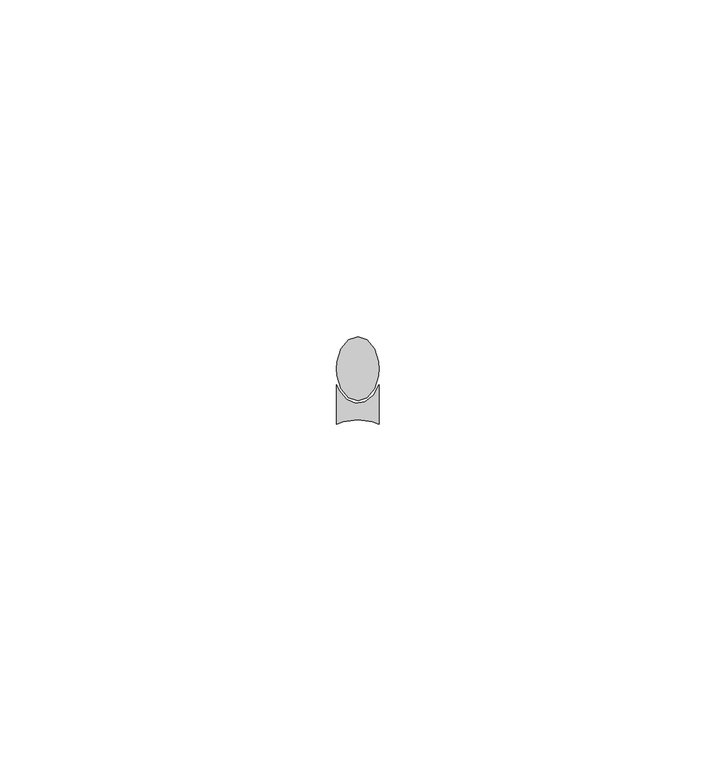
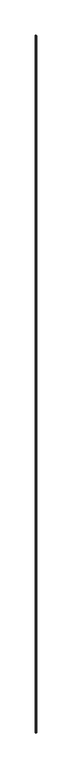
"""IFC4 building model written with IfcOpenShell, lengths in millimetres: proxy geometry, Generic Models 11:Generic Models 1:306267:Generic Models 1:306267 : Generic Models 11:Generic Models 1:306267:300405:Generic Models 1:306267:Generic Models 1:306267 : Generic Models 11:Generic Models 1:306267:300405 : Generic Models 11:Generic Models 1:306267:Generic Models 1:306267 : Generic Models 11:Generic Models 1:306267:300405:13 : Generic Models 11:Generic Models 1:306267:Generic Models 1:306267 : Generic Models 11:Generic Models 1:306267:300405:Generic Models 1:306267:Generic Models 1:306267 : Generic Models 11:Generic Models 1:306267:300405 : Generic Models 11:Generic Models 1:306267:Generic Models 1:306267 : Generic Models 11:Generic Models 1:306267:300405:300182."""

from ifc_helpers import new_model, si_unit, origin, origin_with_axes, place, context, project, spatial, polyline, outline, extrude, source, transform, mapped, element, save


def generic_models_64d3e4db(model_context):
    return source(origin(), model_context, "Body", "SweptSolid", [
        extrude(outline(polyline([(593733.5341431, -579092.0005286), (593732.429409, -579090.6790346), (593731.8163278, -579088.7694203), (593731.7367239, -579087.7096644), (593731.8163278, -579086.6499084), (593732.429409, -579084.7402942), (593733.5341431, -579083.4188002), (593734.9117239, -579082.9471644), (593736.2893048, -579083.4188002), (593737.3940389, -579084.7402942), (593738.0071201, -579086.6499084), (593738.0867239, -579087.7096644), (593738.0071201, -579088.7694203), (593737.3940389, -579090.6790346), (593736.2893048, -579092.0005286), (593734.9117239, -579092.4721644), (593733.5341431, -579092.0005286)])), origin_with_axes(), (0.0, 0.0, 1.0), 6064.4581746),
        extrude(outline(polyline([(593737.1209607, -579095.5639755), (593734.9117239, -579095.2502894), (593732.7024872, -579095.5639755), (593731.7367239, -579095.9413841), (593731.7367239, -579090.073292), (593732.1230415, -579090.9335729), (593733.206527, -579092.2431481), (593734.5567747, -579092.8435016), (593735.962551, -579092.6407137), (593737.2039351, -579091.6665087), (593738.0867239, -579090.073292), (593738.0867239, -579095.9413841), (593737.1209607, -579095.5639755)])), origin_with_axes(), (0.0, 0.0, 1.0), 6062.9878028),
    ])


if __name__ == "__main__":
    model = new_model("IFC4")
    model_context = context("Model", 3, world=origin())
    ifc_project = project(units=[si_unit("LENGTHUNIT", "METRE", prefix="MILLI")], contexts=[model_context])
    site = spatial("IfcSite", under=ifc_project)
    building = spatial("IfcBuilding", under=site)
    placement = place(None, origin())
    generic_models_shape = generic_models_64d3e4db(model_context)
    element("IfcBuildingElementProxy", 1, Name="Generic Models 11:Generic Models 1:306267:Generic Models 1:306267 : Generic Models 11:Generic Models 1:306267:300405:Generic Models 1:306267:Generic Models 1:306267 : Generic Models 11:Generic Models 1:306267:300405 : Generic Models 11:Generic Models 1:306267:Generic Models 1:306267 : Generic Models 11:Generic Models 1:306267:300405:13 : Generic Models 11:Generic Models 1:306267:Generic Models 1:306267 : Generic Models 11:Generic Models 1:306267:300405:Generic Models 1:306267:Generic Models 1:306267 : Generic Models 11:Generic Models 1:306267:300405 : Generic Models 11:Generic Models 1:306267:Generic Models 1:306267 : Generic Models 11:Generic Models 1:306267:300405:300182", ObjectType="Generic Models 11:Generic Models 1:306267:Generic Models 1:306267 : Generic Models 11:Generic Models 1:306267:300405:Generic Models 1:306267:Generic Models 1:306267 : Generic Models 11:Generic Models 1:306267:300405 : Generic Models 11:Generic Models 1:306267:Generic Models 1:306267 : Generic Models 11:Generic Models 1:306267:300405:13 : Generic Models 11:Generic Models 1:306267:Generic Models 1:306267 : Generic Models 11:Generic Models 1:306267:300405:Generic Models 1:306267:Generic Models 1:306267 : Generic Models 11:Generic Models 1:306267:300405 : Generic Models 11:Generic Models 1:306267:Generic Models 1:306267 : Generic Models 11:Generic Models 1:306267:300405:300182", at=placement, inside=building, context=model_context, shape_type="MappedRepresentation", body=[
        mapped(generic_models_shape, transform((0.0, 0.0, 0.0), x_axis=(1.0, 0.0, 0.0), y_axis=(0.0, 1.0, 0.0), z_axis=(0.0, 0.0, 1.0))),
    ])
    save(model, "model.ifc")

# Revit data of these elements
# Type "Generic Models 11:Generic Models 1:306267:Generic Models 1:306267 : Generic Models 11:Generic Models 1:306267:300405:Generic Models 1:306267:Generic Models 1:306267 : Generic Models 11:Generic Models 1:306267:300405 : Generic Models 11:Generic Models 1:306267:Generic Models 1:306267 : Generic Models 11:Generic Models 1:306267:300405:13 : Generic Models 11:Generic Models 1:306267:Generic Models 1:306267 : Generic Models 11:Generic Models 1:306267:300405:Generic Models 1:306267:Generic Models 1:306267 : Generic Models 11:Generic Models 1:306267:300405 : Generic Models 11:Generic Models 1:306267:Generic Models 1:306267 : Generic Models 11:Generic Models 1:306267:300405:300182"
#   NameOverride = "Generic Models 11:Generic Models 1:306267:Generic Models 1:306267 : Generic Models 11:Generic Models 1:306267:300405:Generic Models 1:306267:Generic Models 1:306267 : Generic Models 11:Generic Models 1:306267:300405 : Generic Models 11:Generic Models 1:306267:Generic Models 1:306267 : Generic Models 11:Generic Models 1:306267:300405:300182"
#   ObjectTypeOverride = "Generic Models 1:306267:Generic Models 1:306267 : Generic Models 11:Generic Models 1:306267:300405 : Generic Models 11:Generic Models 1:306267:Generic Models 1:306267 : Generic Models 11:Generic Models 1:306267:300405"
#   Reference = "Generic Models 1"
#   Tag = "300182"
# Element 1 (IfcBuildingElementProxy, "Generic Models 11:Generic Models 1:306267:Generic Models 1:306267 : Generic Models 11:Generic Models 1:306267:300405:Generic Models 1:306267:Generic Models 1:306267 : Generic Models 11:Generic Models 1:306267:300405 : Generic Models 11:Generic Models 1:306267:Generic Models 1:306267 : Generic Models 11:Generic Models 1:306267:300405:13 : Generic Models 11:Generic Models 1:306267:Generic Models 1:306267 : Generic Models 11:Generic Models 1:306267:300405:Generic Models 1:306267:Generic Models 1:306267 : Generic Models 11:Generic Models 1:306267:300405 : Generic Models 11:Generic Models 1:306267:Generic Models 1:306267 : Generic Models 11:Generic Models 1:306267:300405:300182")
#   Materials on its faces: "SEALANT & BACKER ROD"
# Materials
#   "SEALANT & BACKER ROD": class "Unassigned", colour RGB 120 120 120, transparency 0, Cost = 0
